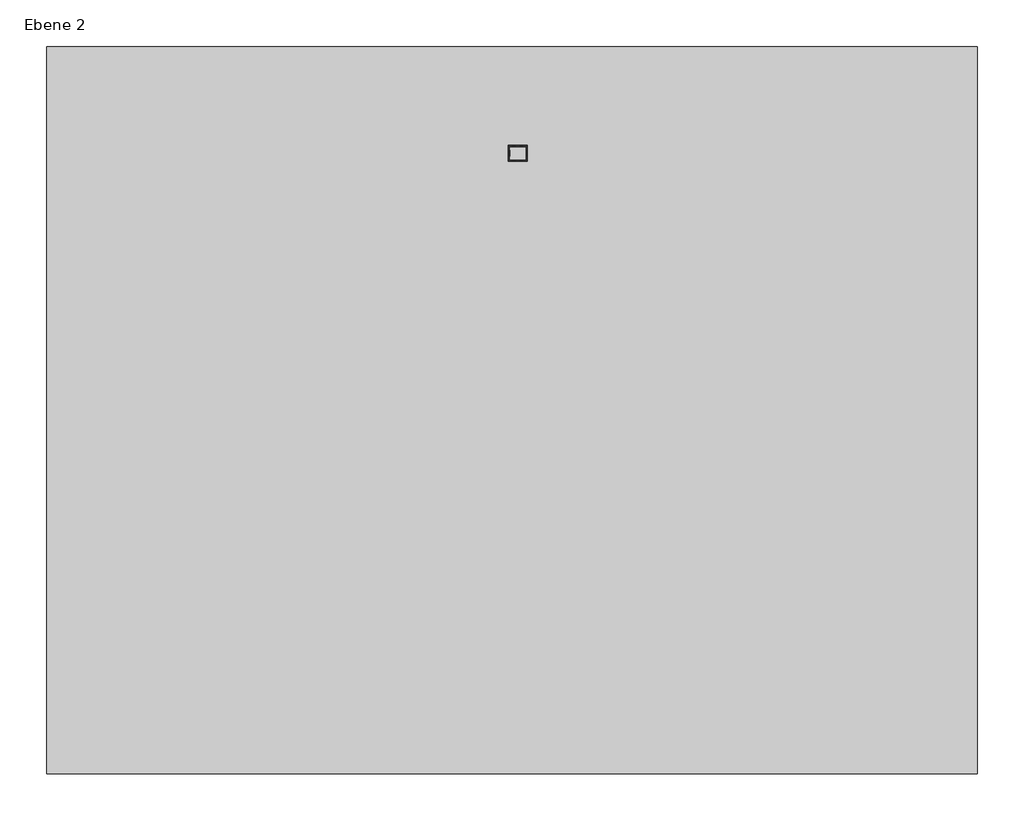
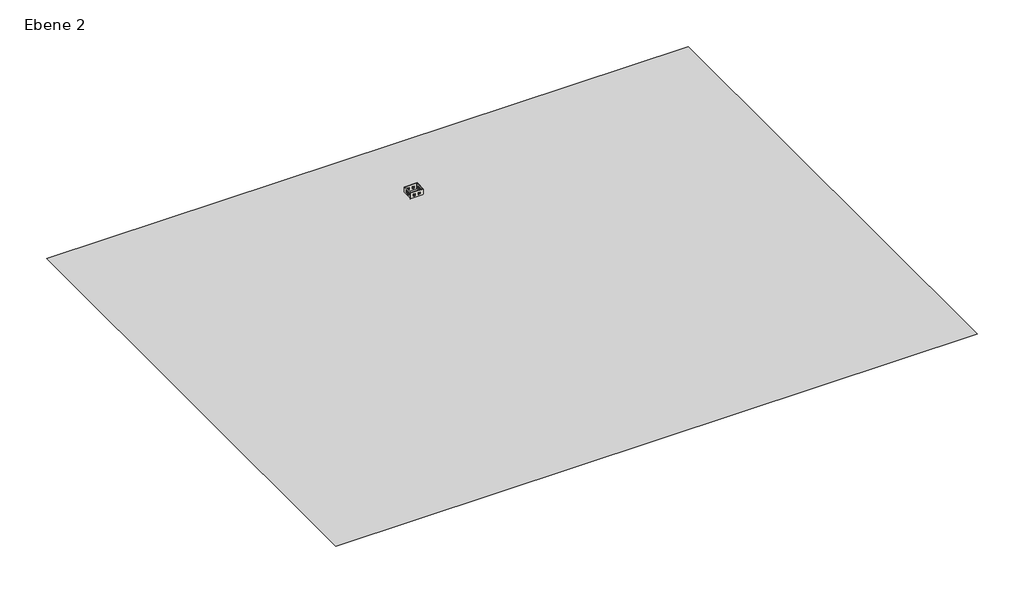
# One storey: 6 windows, 4 walls, 1 proxy.
"""IFC4 building model written with IfcOpenShell, lengths in millimetres."""

import ifcopenshell
import ifcopenshell.guid

model = None  # the IFC model being written
_history = None  # IfcOwnerHistory: only IFC2X3 demands one
_inside = {}  # id of a spatial element -> (the spatial element, [elements in it])
_under = {}  # id of a project, library or spatial element -> (it, [spatial elements below it])
_declared = {}  # id of a project -> (the project, [libraries it declares])
_typed = {}  # id of a type object -> (the type object, [elements of that type])
_made_of = {}  # id of a material, layer set ... -> (it, [elements and type objects made of it])


def new_model(schema):
    """Start an empty IFC model of exactly this schema.

    Asked for "IFC4X3", IfcOpenShell would pick the latest addendum, in which some entities
    have other attributes; the version numbers below select the first issue.
    IFC2X3 requires an IfcOwnerHistory on every rooted entity: one is made here for all.
    """
    global model, _history
    if schema == "IFC4X3":
        model = ifcopenshell.file(schema_version=(4, 3, 0, 0))
    else:
        model = ifcopenshell.file(schema=schema)
    _inside.clear()
    _under.clear()
    _declared.clear()
    _typed.clear()
    _made_of.clear()
    _history = None
    if model.schema == "IFC2X3":
        org = make("IfcOrganization", Name="unknown")
        user = make(
            "IfcPersonAndOrganization",
            ThePerson=make("IfcPerson", FamilyName="unknown"),
            TheOrganization=org,
        )
        app = make(
            "IfcApplication",
            ApplicationDeveloper=org,
            Version="unknown",
            ApplicationFullName="unknown",
            ApplicationIdentifier="unknown",
        )
        _history = make(
            "IfcOwnerHistory",
            OwningUser=user,
            OwningApplication=app,
            ChangeAction="ADDED",
            CreationDate=0,
        )
    return model


def make(cls, **values):
    """One entity of the class cls with the attributes given. An attribute that is None is left unset."""
    return model.create_entity(
        cls, **{name: value for name, value in values.items() if value is not None}
    )


def rooted(cls, **values):
    """An entity with a GlobalId (a new one), such as an element, a storey or a relation."""
    return make(cls, GlobalId=ifcopenshell.guid.new(), OwnerHistory=_history, **values)


def si_unit(unit_type, name, prefix=None):
    """IfcSIUnit, for example si_unit("LENGTHUNIT", "METRE", prefix="MILLI")."""
    return make("IfcSIUnit", UnitType=unit_type, Prefix=prefix, Name=name)


def assignment(units):
    """IfcUnitAssignment: the units of a project."""
    return None if units is None else make("IfcUnitAssignment", Units=units)


def point(xyz):
    """IfcCartesianPoint."""
    return None if xyz is None else make("IfcCartesianPoint", Coordinates=xyz)


def direction(xyz):
    """IfcDirection."""
    return None if xyz is None else make("IfcDirection", DirectionRatios=xyz)


def frame(location, z_axis=None, x_axis=None):
    """IfcAxis2Placement3D, a coordinate frame: its origin and axes. An axis left out is left unset."""
    return make(
        "IfcAxis2Placement3D",
        Location=point(location),
        Axis=direction(z_axis),
        RefDirection=direction(x_axis),
    )


def origin():
    """The frame at (0, 0, 0) with its axes left unset."""
    return frame((0.0, 0.0, 0.0))


def place(relative_to, where):
    """IfcLocalPlacement: puts the frame where relative to a parent placement (None: the world)."""
    return make(
        "IfcLocalPlacement", PlacementRelTo=relative_to, RelativePlacement=where
    )


def context(
    kind, dimensions, precision=None, world=None, true_north=None, identifier=None
):
    """IfcGeometricRepresentationContext, for example the 3D "Model" context."""
    return make(
        "IfcGeometricRepresentationContext",
        ContextIdentifier=identifier,
        ContextType=kind,
        CoordinateSpaceDimension=dimensions,
        Precision=precision,
        WorldCoordinateSystem=world,
        TrueNorth=true_north,
    )


def project(units=None, contexts=None):
    """IfcProject with its units and contexts."""
    return rooted(
        "IfcProject",
        Name="project",
        RepresentationContexts=contexts,
        UnitsInContext=assignment(units),
    )


def spatial(cls, under=None, at=None, **own):
    """A site, building, storey or space (cls), placed at a placement, below another one or the project."""
    s = rooted(cls, ObjectPlacement=at, **own)
    if under is not None:
        _under.setdefault(under.id(), (under, []))[1].append(s)
    return s


def polyline(points):
    """IfcPolyline through the points."""
    return make("IfcPolyline", Points=[point(p) for p in points])


def point_list(points):
    """IfcCartesianPointList2D or 3D."""
    cls = (
        "IfcCartesianPointList2D" if len(points[0]) == 2 else "IfcCartesianPointList3D"
    )
    return make(cls, CoordList=points)


def outline(outer, holes=None, kind="AREA"):
    """IfcArbitraryClosedProfileDef: a profile drawn as a closed curve; with holes, ...WithVoids."""
    if holes is None:
        return make("IfcArbitraryClosedProfileDef", ProfileType=kind, OuterCurve=outer)
    return make(
        "IfcArbitraryProfileDefWithVoids",
        ProfileType=kind,
        OuterCurve=outer,
        InnerCurves=holes,
    )


def extrude(swept, where, along, depth):
    """IfcExtrudedAreaSolid: the profile swept, set in the frame where, extruded along a direction by depth."""
    return make(
        "IfcExtrudedAreaSolid",
        SweptArea=swept,
        Position=where,
        ExtrudedDirection=direction(along),
        Depth=depth,
    )


def faces_of(points, faces, orient=None, outer=None):
    """IfcFace entities. A face is a list of loops; a loop is a list of indices into points, from 0.

    orient and outer hold one flag for each loop. By default every Orientation is true, the
    first loop of a face is its IfcFaceOuterBound and the others are IfcFaceBound.
    """
    made = []
    for i, loops in enumerate(faces):
        bounds = []
        for j, loop in enumerate(loops):
            is_outer = j == 0 if outer is None else outer[i][j]
            bounds.append(
                make(
                    "IfcFaceOuterBound" if is_outer else "IfcFaceBound",
                    Bound=make("IfcPolyLoop", Polygon=[points[k] for k in loop]),
                    Orientation=True if orient is None else orient[i][j],
                )
            )
        made.append(make("IfcFace", Bounds=bounds))
    return made


def faceted_brep(points, faces, orient=None, outer=None, voids=None):
    """IfcFacetedBrep: a solid bounded by flat faces; with voids (closed shells), ...WithVoids."""
    shared = [point(p) for p in points]
    hull = make("IfcClosedShell", CfsFaces=faces_of(shared, faces, orient, outer))
    if voids is None:
        return make("IfcFacetedBrep", Outer=hull)
    return make(
        "IfcFacetedBrepWithVoids",
        Outer=hull,
        Voids=[
            make(cls, CfsFaces=faces_of(shared, fs, o, b)) for cls, fs, o, b in voids
        ],
    )


def triangles(points, corners, closed=None, point_numbers=None):
    """IfcTriangulatedFaceSet: each triangle names its three corners, points numbered from 1."""
    return make(
        "IfcTriangulatedFaceSet",
        Coordinates=point_list(points),
        Closed=closed,
        CoordIndex=corners,
        PnIndex=point_numbers,
    )


def shape(context_of_items, identifier, shape_type, items):
    """IfcShapeRepresentation: the items that make up one representation, for example the "Body"."""
    return make(
        "IfcShapeRepresentation",
        ContextOfItems=context_of_items,
        RepresentationIdentifier=identifier,
        RepresentationType=shape_type,
        Items=items,
    )


def source(mapping_origin, context_of_items, identifier, shape_type, items):
    """IfcRepresentationMap: a shape defined once, which mapped items show again and again."""
    return make(
        "IfcRepresentationMap",
        MappingOrigin=mapping_origin,
        MappedRepresentation=shape(context_of_items, identifier, shape_type, items),
    )


def transform(
    local_origin,
    x_axis=None,
    y_axis=None,
    z_axis=None,
    scale=None,
    scale2=None,
    scale3=None,
    uniform=True,
):
    """IfcCartesianTransformationOperator3D, or its non-uniform kind. x_axis, y_axis, z_axis: its Axis1, 2, 3."""
    if uniform:
        return make(
            "IfcCartesianTransformationOperator3D",
            Axis1=direction(x_axis),
            Axis2=direction(y_axis),
            LocalOrigin=point(local_origin),
            Scale=scale,
            Axis3=direction(z_axis),
        )
    return make(
        "IfcCartesianTransformationOperator3DnonUniform",
        Axis1=direction(x_axis),
        Axis2=direction(y_axis),
        LocalOrigin=point(local_origin),
        Scale=scale,
        Axis3=direction(z_axis),
        Scale2=scale2,
        Scale3=scale3,
    )


def mapped(mapping_source, mapping_target):
    """IfcMappedItem: shows the shape of a source again, moved by a transform."""
    return make(
        "IfcMappedItem", MappingSource=mapping_source, MappingTarget=mapping_target
    )


def made_of(thing, what):
    """Note that an element or type object is made of a material, layer set ...; save() writes the relation."""
    if what is not None:
        _made_of.setdefault(what.id(), (what, []))[1].append(thing)
    return thing


def element(
    cls,
    number,
    at=None,
    inside=None,
    cuts=None,
    type_object=None,
    material=None,
    context=None,
    identifier="Body",
    shape_type=None,
    held_by="IfcProductDefinitionShape",
    body=None,
    shapes=None,
    **own,
):
    """One element of the class cls, such as IfcWall. Its Tag is "e" and its number.

    at: its placement. inside: the storey or other place that contains it. cuts: it is an
    opening in that element (IfcRelVoidsElement). A single representation is given by context,
    identifier, shape_type and body (its items); several are given by shapes. held_by: the class
    of the entity that holds the representations. save() writes the other relations.
    """
    e = rooted(cls, Tag="e%d" % number, ObjectPlacement=at, **own)
    if body is not None:
        shapes = [shape(context, identifier, shape_type, body)]
    if shapes is not None:
        e.Representation = make(held_by, Representations=shapes)
    if inside is not None:
        _inside.setdefault(inside.id(), (inside, []))[1].append(e)
    if cuts is not None:
        rooted(
            "IfcRelVoidsElement", RelatingBuildingElement=cuts, RelatedOpeningElement=e
        )
    if type_object is not None:
        _typed.setdefault(type_object.id(), (type_object, []))[1].append(e)
    return made_of(e, material)


def aggregate(whole, parts):
    """IfcRelAggregates: a whole, such as a stair, and the parts it consists of."""
    return rooted("IfcRelAggregates", RelatingObject=whole, RelatedObjects=parts)


def save(model, path):
    """Write the relations noted so far, then the file.

    IfcRelAggregates (storeys below a building ...), IfcRelContainedInSpatialStructure (elements
    in a storey), IfcRelDefinesByType, IfcRelAssociatesMaterial and IfcRelDeclares: one each for
    every whole, place, type object, material and project.
    """
    for whole, parts in _under.values():
        aggregate(whole, parts)
    for where, things in _inside.values():
        rooted(
            "IfcRelContainedInSpatialStructure",
            RelatedElements=things,
            RelatingStructure=where,
        )
    for kind, things in _typed.values():
        rooted("IfcRelDefinesByType", RelatedObjects=things, RelatingType=kind)
    for what, things in _made_of.values():
        rooted("IfcRelAssociatesMaterial", RelatedObjects=things, RelatingMaterial=what)
    for by, libraries in _declared.values():
        rooted("IfcRelDeclares", RelatingContext=by, RelatedDefinitions=libraries)
    model.write(path)


def fenster_1_flg_variabel_fenster_1_flg_variabel_3_8a378bad(model_context):
    return source(origin(), model_context, "Body", "SolidModel", [
        extrude(outline(polyline([(2010.0, 505.0), (2010.0, -505.0), (1000.0, -505.0), (1000.0, 505.0), (2010.0, 505.0)]), holes=[polyline([(1930.0, 445.0), (1080.0, 445.0), (1080.0, -445.0), (1930.0, -445.0), (1930.0, 445.0)])]), frame((0.0, 40.0, 0.0), z_axis=(0.0, 1.0, 0.0), x_axis=(0.0, 0.0, 1.0)), (0.0, 0.0, 1.0), 60.0),
        faceted_brep([(475.0, 40.0, 1960.0), (475.0, 10.0, 1960.0), (475.0, 10.0, 1050.0), (475.0, 40.0, 1050.0), (-475.0, 10.0, 1960.0), (-475.0, 10.0, 1050.0), (415.0, 10.0, 1110.0), (-415.0, 10.0, 1110.0), (-415.0, 10.0, 1900.0), (415.0, 10.0, 1900.0), (-475.0, 40.0, 1050.0), (-475.0, 40.0, 1960.0), (445.0, 40.0, 1930.0), (-445.0, 40.0, 1930.0), (-445.0, 40.0, 1080.0), (445.0, 40.0, 1080.0), (445.0, 70.0, 1930.0), (445.0, 70.0, 1080.0), (-445.0, 70.0, 1080.0), (-445.0, 70.0, 1930.0), (415.0, 70.0, 1900.0), (-415.0, 70.0, 1900.0), (-415.0, 70.0, 1110.0), (415.0, 70.0, 1110.0)], [[[0, 1, 2, 3]], [[1, 4, 5, 2], [6, 7, 8, 9]], [[3, 2, 5, 10]], [[3, 10, 11, 0], [12, 13, 14, 15]], [[16, 12, 15, 17]], [[17, 15, 14, 18]], [[17, 18, 19, 16], [20, 21, 22, 23]], [[9, 20, 23, 6]], [[6, 23, 22, 7]], [[10, 5, 4, 11]], [[18, 14, 13, 19]], [[7, 22, 21, 8]], [[11, 4, 1, 0]], [[19, 13, 12, 16]], [[8, 21, 20, 9]]]),
        extrude(outline(polyline([(-505.0, -210.0), (-505.0, 40.0), (505.0, 40.0), (505.0, -210.0), (-505.0, -210.0)])), frame((0.0, 0.0, 1005.0), z_axis=(0.0, 0.0, 1.0), x_axis=(1.0, 0.0, 0.0)), (0.0, 0.0, 1.0), 15.0),
        extrude(outline(polyline([(110.0221543, 1020.0), (210.0, 1000.0), (210.0, 990.0), (208.0, 990.0), (208.0, 998.3604634), (109.8240723, 1018.0), (100.0, 1018.0), (100.0, 1020.0), (110.0221543, 1020.0)])), frame((-505.0, 0.0, 0.0), z_axis=(1.0, 0.0, 0.0), x_axis=(0.0, 1.0, 0.0)), (0.0, 0.0, 1.0), 1010.0),
        extrude(outline(polyline([(415.0, 25.0), (-415.0, 25.0), (-415.0, 55.0), (415.0, 55.0), (415.0, 25.0)])), frame((0.0, 0.0, 1110.0), z_axis=(0.0, 0.0, 1.0), x_axis=(1.0, 0.0, 0.0)), (0.0, 0.0, 1.0), 790.0),
    ])


def fenster_2_flg_variabel_fenster_2_flg_variabel_3_03287464(model_context):
    return source(origin(), model_context, "Body", "SolidModel", [
        extrude(outline(polyline([(60.0, -5.0), (915.0, -5.0), (915.0, -35.0), (60.0, -35.0), (60.0, -5.0)])), frame((0.0, 0.0, 1110.0), z_axis=(0.0, 0.0, 1.0), x_axis=(1.0, 0.0, 0.0)), (0.0, 0.0, 1.0), 1040.0),
        extrude(outline(polyline([(-915.0, -5.0), (-60.0, -5.0), (-60.0, -35.0), (-915.0, -35.0), (-915.0, -5.0)])), frame((0.0, 0.0, 1110.0), z_axis=(0.0, 0.0, 1.0), x_axis=(1.0, 0.0, 0.0)), (0.0, 0.0, 1.0), 1040.0),
        extrude(outline(polyline([(-1005.0, -210.0), (-1005.0, -20.0), (1005.0, -20.0), (1005.0, -210.0), (-1005.0, -210.0)])), frame((0.0, 0.0, 1005.0), z_axis=(0.0, 0.0, 1.0), x_axis=(1.0, 0.0, 0.0)), (0.0, 0.0, 1.0), 15.0),
        extrude(outline(polyline([(50.0221543, 1020.0), (210.0, 1000.0), (210.0, 990.0), (208.0, 990.0), (208.0, 998.3604634), (49.8240723, 1018.0), (40.0, 1018.0), (40.0, 1020.0), (50.0221543, 1020.0)])), frame((-1005.0, 0.0, 0.0), z_axis=(1.0, 0.0, 0.0), x_axis=(0.0, 1.0, 0.0)), (0.0, 0.0, 1.0), 2010.0),
        extrude(outline(polyline([(30.0, -20.0), (-30.0, -20.0), (-30.0, 40.0), (30.0, 40.0), (30.0, -20.0)])), frame((0.0, 0.0, 1080.0), z_axis=(0.0, 0.0, 1.0), x_axis=(1.0, 0.0, 0.0)), (0.0, 0.0, 1.0), 1100.0),
        extrude(outline(polyline([(2260.0, -1005.0), (1000.0, -1005.0), (1000.0, 1005.0), (2260.0, 1005.0), (2260.0, -1005.0)]), holes=[polyline([(2180.0, -945.0), (2180.0, 945.0), (1080.0, 945.0), (1080.0, -945.0), (2180.0, -945.0)])]), frame((0.0, -20.0, 0.0), z_axis=(0.0, 1.0, 0.0), x_axis=(0.0, 0.0, 1.0)), (0.0, 0.0, 1.0), 60.0),
        faceted_brep([(-945.0, -20.0, 1080.0), (-945.0, 10.0, 1080.0), (-30.0, 10.0, 1080.0), (-30.0, -20.0, 1080.0), (-30.0, 10.0, 2180.0), (-30.0, -20.0, 2180.0), (-945.0, 10.0, 2180.0), (-60.0, 10.0, 2150.0), (-915.0, 10.0, 2150.0), (-915.0, 10.0, 1110.0), (-60.0, 10.0, 1110.0), (0.0, -20.0, 1050.0), (-975.0, -20.0, 1050.0), (-975.0, -20.0, 2210.0), (0.0, -20.0, 2210.0), (-945.0, -20.0, 2180.0), (-975.0, -50.0, 1050.0), (0.0, -50.0, 1050.0), (0.0, -50.0, 2210.0), (-975.0, -50.0, 2210.0), (-60.0, -50.0, 1110.0), (-915.0, -50.0, 1110.0), (-915.0, -50.0, 2150.0), (-60.0, -50.0, 2150.0)], [[[0, 1, 2, 3]], [[3, 2, 4, 5]], [[2, 1, 6, 4], [7, 8, 9, 10]], [[11, 12, 13, 14], [5, 15, 0, 3]], [[16, 12, 11, 17]], [[17, 11, 14, 18]], [[18, 19, 16, 17], [20, 21, 22, 23]], [[9, 21, 20, 10]], [[10, 20, 23, 7]], [[15, 6, 1, 0]], [[19, 13, 12, 16]], [[8, 22, 21, 9]], [[5, 4, 6, 15]], [[18, 14, 13, 19]], [[7, 23, 22, 8]]]),
        faceted_brep([(30.0, -20.0, 1080.0), (30.0, 10.0, 1080.0), (945.0, 10.0, 1080.0), (945.0, -20.0, 1080.0), (945.0, 10.0, 2180.0), (945.0, -20.0, 2180.0), (30.0, 10.0, 2180.0), (915.0, 10.0, 2150.0), (60.0, 10.0, 2150.0), (60.0, 10.0, 1110.0), (915.0, 10.0, 1110.0), (975.0, -20.0, 1050.0), (0.0, -20.0, 1050.0), (0.0, -20.0, 2210.0), (975.0, -20.0, 2210.0), (30.0, -20.0, 2180.0), (0.0, -50.0, 1050.0), (975.0, -50.0, 1050.0), (975.0, -50.0, 2210.0), (0.0, -50.0, 2210.0), (915.0, -50.0, 1110.0), (60.0, -50.0, 1110.0), (60.0, -50.0, 2150.0), (915.0, -50.0, 2150.0)], [[[0, 1, 2, 3]], [[3, 2, 4, 5]], [[2, 1, 6, 4], [7, 8, 9, 10]], [[11, 12, 13, 14], [5, 15, 0, 3]], [[16, 12, 11, 17]], [[17, 11, 14, 18]], [[18, 19, 16, 17], [20, 21, 22, 23]], [[9, 21, 20, 10]], [[10, 20, 23, 7]], [[15, 6, 1, 0]], [[19, 13, 12, 16]], [[8, 22, 21, 9]], [[5, 4, 6, 15]], [[18, 14, 13, 19]], [[7, 23, 22, 8]]]),
    ])


model = new_model("IFC4")

# Units and contexts
model_context = context("Model", 3, world=origin())
ifc_project = project(units=[si_unit("LENGTHUNIT", "METRE", prefix="MILLI")], contexts=[model_context])

# Site, building, storey
site = spatial("IfcSite", under=ifc_project)
building = spatial("IfcBuilding", under=site)
storey = spatial("IfcBuildingStorey", under=building, Name="Ebene 2", Elevation=6000.0)

# Proxy
placement = place(None, origin())
element("IfcBuildingElementProxy", 1, Name="Building Element Proxy", at=placement, inside=storey, context=model_context, shape_type="Tessellation", body=[
    triangles([(-160331.1996094, -208151.4062988, 6096.0), (154493.6024414, -208151.4062988, 6096.0), (154493.6024414, 37859.0007568, 6096.0), (-160331.1996094, 37859.0007568, 6096.0)], [[4, 1, 2], [2, 3, 4]], closed=False),
])

# Walls
element("IfcWall", 2, ObjectType="MW 24.0 WD 12.0", at=placement, inside=storey, context=model_context, shape_type="Brep", body=[
    faceted_brep([(-3766.4979049, 4044.3692517, 6000.0), (1873.5020951, 4044.3692517, 6000.0), (1873.5020951, 4044.3692517, 9000.0), (-3766.4979049, 4044.3692517, 9000.0), (673.5020951, 4044.3692517, 7000.0), (-336.4979049, 4044.3692517, 7000.0), (-336.4979049, 4044.3692517, 8010.0), (673.5020951, 4044.3692517, 8010.0), (-1756.4979049, 4044.3692517, 7000.0), (-2766.4979049, 4044.3692517, 7000.0), (-2766.4979049, 4044.3692517, 8010.0), (-1756.4979049, 4044.3692517, 8010.0), (-4126.4979049, 4404.3692517, 6000.0), (-4126.4979049, 4404.3692517, 9000.0), (2233.5020951, 4404.3692517, 9000.0), (2233.5020951, 4404.3692517, 6000.0), (673.5020951, 4404.3692517, 7000.0), (673.5020951, 4404.3692517, 8010.0), (-336.4979049, 4404.3692517, 8010.0), (-336.4979049, 4404.3692517, 7000.0), (-1756.4979049, 4404.3692517, 7000.0), (-1756.4979049, 4404.3692517, 8010.0), (-2766.4979049, 4404.3692517, 8010.0), (-2766.4979049, 4404.3692517, 7000.0)], [[[0, 1, 2, 3], [4, 5, 6, 7], [8, 9, 10, 11]], [[12, 13, 14, 15], [16, 17, 18, 19], [20, 21, 22, 23]], [[1, 0, 12, 15]], [[3, 2, 14, 13]], [[2, 1, 15, 14]], [[0, 3, 13, 12]], [[17, 16, 4, 7]], [[18, 17, 7, 6]], [[19, 18, 6, 5]], [[16, 19, 5, 4]], [[21, 20, 8, 11]], [[22, 21, 11, 10]], [[23, 22, 10, 9]], [[20, 23, 9, 8]]]),
])
element("IfcWall", 3, ObjectType="MW 24.0 WD 12.0", at=placement, inside=storey, context=model_context, shape_type="Brep", body=[
    faceted_brep([(1873.5020951, 4044.3692517, 6000.0), (1873.5020951, -595.6307483, 6000.0), (1873.5020951, -595.6307483, 9000.0), (1873.5020951, 4044.3692517, 9000.0), (1873.5020951, 719.3692517, 7000.0), (1873.5020951, 2729.3692517, 7000.0), (1873.5020951, 2729.3692517, 8260.0), (1873.5020951, 719.3692517, 8260.0), (2233.5020951, 4404.3692517, 6000.0), (2233.5020951, 4404.3692517, 9000.0), (2233.5020951, -955.6307483, 9000.0), (2233.5020951, -955.6307483, 6000.0), (2233.5020951, 719.3692517, 7000.0), (2233.5020951, 719.3692517, 8260.0), (2233.5020951, 2729.3692517, 8260.0), (2233.5020951, 2729.3692517, 7000.0)], [[[0, 1, 2, 3], [4, 5, 6, 7]], [[8, 9, 10, 11], [12, 13, 14, 15]], [[1, 0, 8, 11]], [[3, 2, 10, 9]], [[0, 3, 9, 8]], [[2, 1, 11, 10]], [[13, 12, 4, 7]], [[14, 13, 7, 6]], [[15, 14, 6, 5]], [[12, 15, 5, 4]]]),
])
element("IfcWall", 4, ObjectType="MW 24.0 WD 12.0", at=placement, inside=storey, context=model_context, shape_type="Brep", body=[
    faceted_brep([(1873.5020951, -595.6307483, 6000.0), (-3766.4979049, -595.6307483, 6000.0), (-3766.4979049, -595.6307483, 9000.0), (1873.5020951, -595.6307483, 9000.0), (-336.4979049, -595.6307483, 7000.0), (673.5020951, -595.6307483, 7000.0), (673.5020951, -595.6307483, 8010.0), (-336.4979049, -595.6307483, 8010.0), (-2766.4979049, -595.6307483, 7000.0), (-1756.4979049, -595.6307483, 7000.0), (-1756.4979049, -595.6307483, 8010.0), (-2766.4979049, -595.6307483, 8010.0), (2233.5020951, -955.6307483, 6000.0), (2233.5020951, -955.6307483, 9000.0), (-4126.4979049, -955.6307483, 9000.0), (-4126.4979049, -955.6307483, 6000.0), (-336.4979049, -955.6307483, 7000.0), (-336.4979049, -955.6307483, 8010.0), (673.5020951, -955.6307483, 8010.0), (673.5020951, -955.6307483, 7000.0), (-2766.4979049, -955.6307483, 7000.0), (-2766.4979049, -955.6307483, 8010.0), (-1756.4979049, -955.6307483, 8010.0), (-1756.4979049, -955.6307483, 7000.0)], [[[0, 1, 2, 3], [4, 5, 6, 7], [8, 9, 10, 11]], [[12, 13, 14, 15], [16, 17, 18, 19], [20, 21, 22, 23]], [[1, 0, 12, 15]], [[3, 2, 14, 13]], [[0, 3, 13, 12]], [[2, 1, 15, 14]], [[17, 16, 4, 7]], [[18, 17, 7, 6]], [[19, 18, 6, 5]], [[16, 19, 5, 4]], [[21, 20, 8, 11]], [[22, 21, 11, 10]], [[23, 22, 10, 9]], [[20, 23, 9, 8]]]),
])
element("IfcWall", 5, ObjectType="MW 24.0 WD 12.0", at=placement, inside=storey, context=model_context, shape_type="Brep", body=[
    faceted_brep([(-3766.4979049, -595.6307483, 6000.0), (-3766.4979049, 4044.3692517, 6000.0), (-3766.4979049, 4044.3692517, 9000.0), (-3766.4979049, -595.6307483, 9000.0), (-3766.4979049, 2729.3692517, 7000.0), (-3766.4979049, 719.3692517, 7000.0), (-3766.4979049, 719.3692517, 8260.0), (-3766.4979049, 2729.3692517, 8260.0), (-4126.4979049, -955.6307483, 6000.0), (-4126.4979049, -955.6307483, 9000.0), (-4126.4979049, 4404.3692517, 9000.0), (-4126.4979049, 4404.3692517, 6000.0), (-4126.4979049, 2729.3692517, 7000.0), (-4126.4979049, 2729.3692517, 8260.0), (-4126.4979049, 719.3692517, 8260.0), (-4126.4979049, 719.3692517, 7000.0)], [[[0, 1, 2, 3], [4, 5, 6, 7]], [[8, 9, 10, 11], [12, 13, 14, 15]], [[1, 0, 8, 11]], [[3, 2, 10, 9]], [[2, 1, 11, 10]], [[0, 3, 9, 8]], [[13, 12, 4, 7]], [[14, 13, 7, 6]], [[15, 14, 6, 5]], [[12, 15, 5, 4]]]),
])

# Windows
fenster_1_flg_variabel_fenster_1_flg_variabel_3_shape = fenster_1_flg_variabel_fenster_1_flg_variabel_3_8a378bad(model_context)
element("IfcWindow", 6, ObjectType="Fenster 1-flg - Variabel : Fenster 1-flg - Variabel 3", at=placement, inside=storey, context=model_context, shape_type="MappedRepresentation", body=[
    mapped(fenster_1_flg_variabel_fenster_1_flg_variabel_3_shape, transform((168.5020951, -775.6307483, 6000.0), x_axis=(1.0, 0.0, 0.0), y_axis=(0.0, 1.0, 0.0), z_axis=(0.0, 0.0, 1.0))),
])
element("IfcWindow", 7, ObjectType="Fenster 1-flg - Variabel : Fenster 1-flg - Variabel 3", at=placement, inside=storey, context=model_context, shape_type="MappedRepresentation", body=[
    mapped(fenster_1_flg_variabel_fenster_1_flg_variabel_3_shape, transform((-2261.4979049, -775.6307483, 6000.0), x_axis=(1.0, 0.0, 0.0), y_axis=(0.0, 1.0, 0.0), z_axis=(0.0, 0.0, 1.0))),
])
element("IfcWindow", 8, ObjectType="Fenster 1-flg - Variabel : Fenster 1-flg - Variabel 3", at=placement, inside=storey, context=model_context, shape_type="MappedRepresentation", body=[
    mapped(fenster_1_flg_variabel_fenster_1_flg_variabel_3_shape, transform((168.5020951, 4224.3692517, 6000.0), x_axis=(-1.0, 0.0, 0.0), y_axis=(0.0, -1.0, 0.0), z_axis=(0.0, 0.0, 1.0))),
])
element("IfcWindow", 9, ObjectType="Fenster 1-flg - Variabel : Fenster 1-flg - Variabel 3", at=placement, inside=storey, context=model_context, shape_type="MappedRepresentation", body=[
    mapped(fenster_1_flg_variabel_fenster_1_flg_variabel_3_shape, transform((-2261.4979049, 4224.3692517, 6000.0), x_axis=(-1.0, 0.0, 0.0), y_axis=(0.0, -1.0, 0.0), z_axis=(0.0, 0.0, 1.0))),
])
fenster_2_flg_variabel_fenster_2_flg_variabel_3_shape = fenster_2_flg_variabel_fenster_2_flg_variabel_3_03287464(model_context)
element("IfcWindow", 10, ObjectType="Fenster 2-flg - Variabel : Fenster 2-flg - Variabel 3", at=placement, inside=storey, context=model_context, shape_type="MappedRepresentation", body=[
    mapped(fenster_2_flg_variabel_fenster_2_flg_variabel_3_shape, transform((2053.5020951, 1724.3692517, 6000.0), x_axis=(0.0, 1.0, 0.0), y_axis=(-1.0, 0.0, 0.0), z_axis=(0.0, 0.0, 1.0))),
])
element("IfcWindow", 11, ObjectType="Fenster 2-flg - Variabel : Fenster 2-flg - Variabel 3", at=placement, inside=storey, context=model_context, shape_type="MappedRepresentation", body=[
    mapped(fenster_2_flg_variabel_fenster_2_flg_variabel_3_shape, transform((-3946.4979049, 1724.3692517, 6000.0), x_axis=(0.0, -1.0, 0.0), y_axis=(1.0, 0.0, 0.0), z_axis=(0.0, 0.0, 1.0))),
])

save(model, "model.ifc")

# Revit data of these elements
# Type "MW 24.0 WD 12.0"
#   Type Comments = "Mehrschaliges Mauerwerk"
#   Description = "Mauerwerk 24.0 cm, Wärmedämmung 12.0 cm"
#   Layers, outside or top first: 0.120 m "Wärmedämmung - hart" (function 3); 0.240 m "Mauerwerk - Ziegel, verputzt" (function 1)
# Type "Fenster 1-flg - Variabel : Fenster 1-flg - Variabel 3"
#   Type Mark = "52"
#   Operation = "SinglePanel"
#   Construction Type Id = "GSP4R"
#   Keynote = "16.05.01"
#   Analytic Construction = "1/8 Zoll Pilkington-Verglasung einfach"
#   Cost = 78.2
#   Visual Light Transmittance = 0.9
#   Höhe oberer  Rahmen = 0.080 m
#   Solar Heat Gain Coefficient = 0.86
#   Tiefe Flügel = 0.060 m
#   Rough Width [instance default] = 1.010 m
#   Rough Height [instance default] = 1.010 m
#   Rahmenhöhe unten = 0.080 m
#   Heat Transfer Coefficient (U) = 6.7069 W/(m²·K)
#   Rahmentiefe = 0.060 m
#   Rahmenbreite = 0.060 m
#   Height [instance default] = 1.010 m
#   Flügelbreite = 0.060 m
#   Einbautiefe (von außen) [instance default] = 0.080 m
#   Width [instance default] = 1.010 m
#   Define Thermal Properties by = 1
#   Öffnungsrichtung oben [instance default] = yes
#   Öffnungsrichtung in Draufsicht anzeigen [instance default] = no
#   Klappflügel [instance default] = no
#   Drehflügel 1 [instance default] = yes
#   Fensterflügel [instance default] = none
#   Innere Fensterbank [instance default] = none
#   Glas [instance default] = none
#   Bild [instance default] = none
#   Äußere Fensterbank [instance default] = none
#   Wall Closure = (empty or 0)
# Type "Fenster 2-flg - Variabel : Fenster 2-flg - Variabel 3"
#   Type Mark = "53"
#   Operation = "DoublePanelVertical"
#   Construction Type Id = "GSP4R"
#   Keynote = "16.05.01"
#   Analytic Construction = "1/8 Zoll Pilkington-Verglasung einfach"
#   Cost = 130.98
#   Visual Light Transmittance = 0.9
#   Solar Heat Gain Coefficient = 0.78
#   Rough Width [instance default] = 2.010 m
#   Rough Height [instance default] = 1.260 m
#   Heat Transfer Coefficient (U) = 3.6886 W/(m²·K)
#   Rahmentiefe = 0.060 m
#   Rahmenhöhe unten = 0.080 m
#   Höhe oberer  Rahmen = 0.080 m
#   Rahmenbreite = 0.060 m
#   Height [instance default] = 1.260 m
#   Tiefe Flügel = 0.060 m
#   Flügelbreite = 0.060 m
#   Einbautiefe (von außen) [instance default] = 0.140 m
#   Width [instance default] = 2.010 m
#   Define Thermal Properties by = 1
#   Öffnungsrichtung oben [instance default] = yes
#   Öffnungsrichtung in Draufsicht anzeigen [instance default] = no
#   Drehflügel 1 [instance default] = yes
#   Bild [instance default] = none
#   Glas [instance default] = none
#   Fensterflügel [instance default] = none
#   Äußere Fensterbank [instance default] = none
#   Innere Fensterbank [instance default] = none
#   Wall Closure = (empty or 0)
# Element 1 (IfcBuildingElementProxy)
#   Comments = "Reference plane: BP_BauGrenze"
#   Material = transparent
#   Phase Created = Phase 1
# Elements 2, 3, 4, 5 (IfcWall, "MW 24.0 WD 12.0")
#   Comments = ""
#   Top Offset = 0.000 m
#   Base Offset = 0.000 m
#   Unconnected Height = 3.000 m
#   wall height = 3.000 m
#   Phase Created = Phase 1
#   Base Constraint = Ebene 2
#   Materials on its faces: "Vorgabe - Wand", "Mauerwerk - Ziegel, verputzt", "Wärmedämmung - hart"
# Element 6 (IfcWindow, "Fenster 1-flg - Variabel : Fenster 1-flg - Variabel 3")
#   Mark = "10"
#   Rough Height = 1.010 m
#   Rough Width = 1.010 m
#   Height = 1.010 m
#   Einbautiefe (von außen) = 0.080 m
#   Width = 1.010 m
#   Öffnungsrichtung oben = yes
#   Öffnungsrichtung in Draufsicht anzeigen = no
#   Klappflügel = no
#   Drehflügel 1 = yes
#   Äußere Fensterbank = none
#   Innere Fensterbank = none
#   Glas = none
#   Fensterflügel = none
#   Bild = none
#   Phase Created = Phase 1
#   Materials on its faces: "Kunststoff - Weiß", "Holz - Birke", "Glas"
# Element 7 (IfcWindow, "Fenster 1-flg - Variabel : Fenster 1-flg - Variabel 3")
#   Mark = "11"
#   Rough Height = 1.010 m
#   Rough Width = 1.010 m
#   Height = 1.010 m
#   Einbautiefe (von außen) = 0.080 m
#   Width = 1.010 m
#   Öffnungsrichtung oben = yes
#   Öffnungsrichtung in Draufsicht anzeigen = no
#   Klappflügel = no
#   Drehflügel 1 = yes
#   Äußere Fensterbank = none
#   Innere Fensterbank = none
#   Glas = none
#   Fensterflügel = none
#   Bild = none
#   Phase Created = Phase 1
#   Materials on its faces: "Kunststoff - Weiß", "Holz - Birke", "Glas"
# Element 8 (IfcWindow, "Fenster 1-flg - Variabel : Fenster 1-flg - Variabel 3")
#   Mark = "12"
#   Rough Height = 1.010 m
#   Rough Width = 1.010 m
#   Height = 1.010 m
#   Einbautiefe (von außen) = 0.080 m
#   Width = 1.010 m
#   Öffnungsrichtung oben = yes
#   Öffnungsrichtung in Draufsicht anzeigen = no
#   Klappflügel = no
#   Drehflügel 1 = yes
#   Äußere Fensterbank = none
#   Innere Fensterbank = none
#   Glas = none
#   Fensterflügel = none
#   Bild = none
#   Phase Created = Phase 1
#   Materials on its faces: "Kunststoff - Weiß", "Holz - Birke", "Glas"
# Element 9 (IfcWindow, "Fenster 1-flg - Variabel : Fenster 1-flg - Variabel 3")
#   Mark = "13"
#   Rough Height = 1.010 m
#   Rough Width = 1.010 m
#   Height = 1.010 m
#   Einbautiefe (von außen) = 0.080 m
#   Width = 1.010 m
#   Öffnungsrichtung oben = yes
#   Öffnungsrichtung in Draufsicht anzeigen = no
#   Klappflügel = no
#   Drehflügel 1 = yes
#   Äußere Fensterbank = none
#   Innere Fensterbank = none
#   Glas = none
#   Fensterflügel = none
#   Bild = none
#   Phase Created = Phase 1
#   Materials on its faces: "Kunststoff - Weiß", "Holz - Birke", "Glas"
# Element 10 (IfcWindow, "Fenster 2-flg - Variabel : Fenster 2-flg - Variabel 3")
#   Mark = "14"
#   Rough Height = 1.260 m
#   Rough Width = 2.010 m
#   Height = 1.260 m
#   Einbautiefe (von außen) = 0.140 m
#   Width = 2.010 m
#   Öffnungsrichtung oben = yes
#   Öffnungsrichtung in Draufsicht anzeigen = no
#   Drehflügel 1 = yes
#   Äußere Fensterbank = none
#   Innere Fensterbank = none
#   Glas = none
#   Fensterflügel = none
#   Bild = none
#   Phase Created = Phase 1
#   Materials on its faces: "Kunststoff - Weiß", "Glas", "Holz - Birke"
# Element 11 (IfcWindow, "Fenster 2-flg - Variabel : Fenster 2-flg - Variabel 3")
#   Mark = "15"
#   Rough Height = 1.260 m
#   Rough Width = 2.010 m
#   Height = 1.260 m
#   Einbautiefe (von außen) = 0.140 m
#   Width = 2.010 m
#   Öffnungsrichtung oben = yes
#   Öffnungsrichtung in Draufsicht anzeigen = no
#   Drehflügel 1 = yes
#   Äußere Fensterbank = none
#   Innere Fensterbank = none
#   Glas = none
#   Fensterflügel = none
#   Bild = none
#   Phase Created = Phase 1
#   Materials on its faces: "Kunststoff - Weiß", "Glas", "Holz - Birke"
# Materials
#   "Wärmedämmung - hart": class "Stuck", colour RGB 255 255 255, transparency 0, Description = "Äußere Oberfläche", Cost = 0
#   "Mauerwerk - Ziegel, verputzt": class "Stuck", colour RGB 247 247 247, transparency 0, Cost = 0
#   "transparent": class "Nicht zugewiesen", colour RGB 0 0 0, transparency 1
#   "Vorgabe - Wand": class "Stuck", colour RGB 128 128 128, transparency 0, Description = "Äußere Oberfläche", Cost = 0
#   "Kunststoff - Weiß": class "Kunststoff", colour RGB 249 249 249, transparency 0, Cost = 0
#   "Holz - Birke": class "Holz", colour RGB 213 164 103, transparency 0, Cost = 0
#   "Glas": class "Glas", colour RGB 0 0 255, transparency 0.75, Comments = "Render-Darstellung nicht aktualisiert ", Cost = 0
